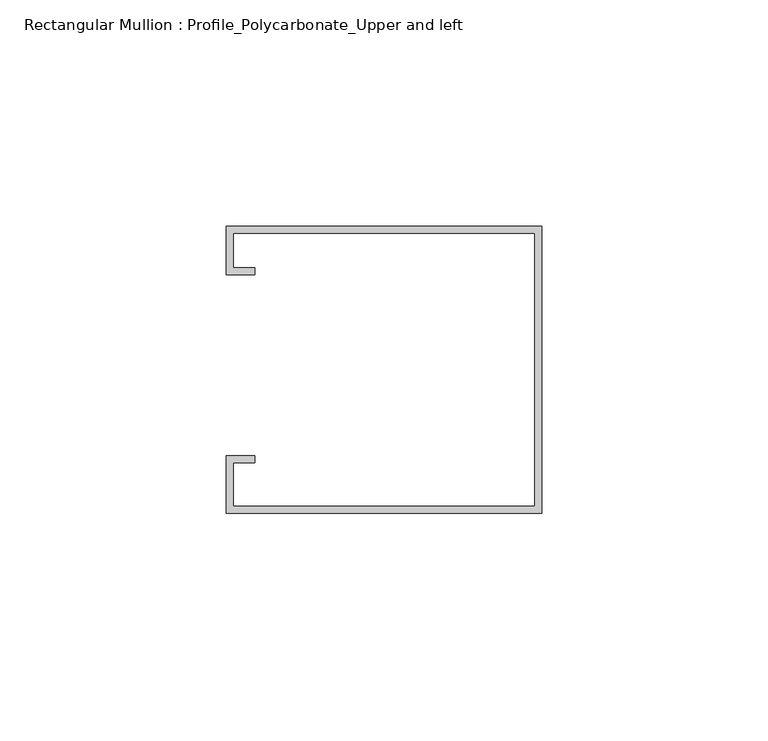
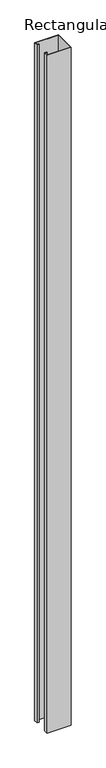
"""IFC4 building model written with IfcOpenShell, lengths in millimetres: member geometry, Rectangular Mullion : Profile_Polycarbonate_Upper and left."""

from ifc_helpers import new_model, si_unit, frame, origin, place, context, project, spatial, polyline, outline, extrude, source, transform, mapped, element, save


def rectangular_mullion_profile_polycarbonate_upper_and_left_984463af(model_context):
    return source(origin(), model_context, "Body", "SweptSolid", [
        extrude(outline(polyline([(0.0, -32.7), (-69.85, -32.7), (-69.85, -20.0), (-63.5, -20.0), (-63.5, -21.5875), (-68.2625, -21.5875), (-68.2625, -31.1125), (-1.5875, -31.1125), (-1.5875, 29.2125), (-68.2625, 29.2125), (-68.2625, 21.5875), (-63.5, 21.5875), (-63.5, 20.0), (-69.85, 20.0), (-69.85, 30.8), (0.0, 30.8), (0.0, -32.7)])), frame((0.0, 0.0, -2090.8202426), z_axis=(0.0, 0.0, 1.0), x_axis=(1.0, 0.0, 0.0)), (0.0, 0.0, 1.0), 2090.8202426),
    ])


if __name__ == "__main__":
    model = new_model("IFC4")
    model_context = context("Model", 3, world=origin())
    ifc_project = project(units=[si_unit("LENGTHUNIT", "METRE", prefix="MILLI")], contexts=[model_context])
    site = spatial("IfcSite", under=ifc_project)
    building = spatial("IfcBuilding", under=site)
    placement = place(None, origin())
    rectangular_mullion_profile_polycarbonate_upper_and_left_shape = rectangular_mullion_profile_polycarbonate_upper_and_left_984463af(model_context)
    element("IfcMember", 1, ObjectType="Rectangular Mullion : Profile_Polycarbonate_Upper and left", at=placement, inside=building, context=model_context, shape_type="MappedRepresentation", body=[
        mapped(rectangular_mullion_profile_polycarbonate_upper_and_left_shape, transform((0.0, 0.0, 0.0), x_axis=(1.0, 0.0, 0.0), y_axis=(0.0, 1.0, 0.0), z_axis=(0.0, 0.0, 1.0))),
    ])
    save(model, "model.ifc")

# Revit data of these elements
# Type "Rectangular Mullion : Profile_Polycarbonate_Upper and left"
#   built-in parameter 1007322 = 0.208333 (stored number, unit not read)
#   built-in parameter 1007321 = 0.00520833 (stored number, unit not read)
#   built-in parameter 1007320 = 0 (stored number, unit not read)
# Element 1 (IfcMember, "Rectangular Mullion : Profile_Polycarbonate_Upper and left")
#   Materials on its faces: "GALVANIZED UNISTRUT P5500, 1 5/8\" X 2 7/16\" OR ALUM. CHANNEL"
# Materials
#   "GALVANIZED UNISTRUT P5500, 1 5/8\" X 2 7/16\" OR ALUM. CHANNEL": class "Metal", colour RGB 244 244 244, transparency 0, Description = "Aluminum 6061", Cost = 0
